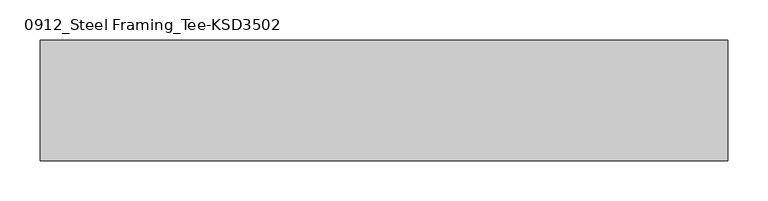
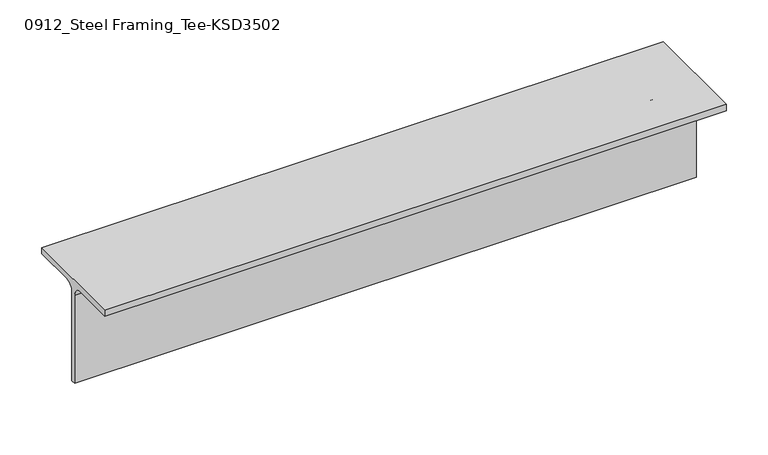
"""IFC4 building model written with IfcOpenShell, lengths in millimetres: member geometry, 0912_Steel Framing_Tee-KSD3502 : H_SB_ASB_CT-150x150x6.5x9."""

import ifcopenshell
import ifcopenshell.guid

model = None  # the IFC model being written
_history = None  # IfcOwnerHistory: only IFC2X3 demands one
_inside = {}  # id of a spatial element -> (the spatial element, [elements in it])
_under = {}  # id of a project, library or spatial element -> (it, [spatial elements below it])
_declared = {}  # id of a project -> (the project, [libraries it declares])
_typed = {}  # id of a type object -> (the type object, [elements of that type])
_made_of = {}  # id of a material, layer set ... -> (it, [elements and type objects made of it])


def new_model(schema):
    """Start an empty IFC model of exactly this schema.

    Asked for "IFC4X3", IfcOpenShell would pick the latest addendum, in which some entities
    have other attributes; the version numbers below select the first issue.
    IFC2X3 requires an IfcOwnerHistory on every rooted entity: one is made here for all.
    """
    global model, _history
    if schema == "IFC4X3":
        model = ifcopenshell.file(schema_version=(4, 3, 0, 0))
    else:
        model = ifcopenshell.file(schema=schema)
    _inside.clear()
    _under.clear()
    _declared.clear()
    _typed.clear()
    _made_of.clear()
    _history = None
    if model.schema == "IFC2X3":
        org = make("IfcOrganization", Name="unknown")
        user = make(
            "IfcPersonAndOrganization",
            ThePerson=make("IfcPerson", FamilyName="unknown"),
            TheOrganization=org,
        )
        app = make(
            "IfcApplication",
            ApplicationDeveloper=org,
            Version="unknown",
            ApplicationFullName="unknown",
            ApplicationIdentifier="unknown",
        )
        _history = make(
            "IfcOwnerHistory",
            OwningUser=user,
            OwningApplication=app,
            ChangeAction="ADDED",
            CreationDate=0,
        )
    return model


def make(cls, **values):
    """One entity of the class cls with the attributes given. An attribute that is None is left unset."""
    return model.create_entity(
        cls, **{name: value for name, value in values.items() if value is not None}
    )


def rooted(cls, **values):
    """An entity with a GlobalId (a new one), such as an element, a storey or a relation."""
    return make(cls, GlobalId=ifcopenshell.guid.new(), OwnerHistory=_history, **values)


def si_unit(unit_type, name, prefix=None):
    """IfcSIUnit, for example si_unit("LENGTHUNIT", "METRE", prefix="MILLI")."""
    return make("IfcSIUnit", UnitType=unit_type, Prefix=prefix, Name=name)


def assignment(units):
    """IfcUnitAssignment: the units of a project."""
    return None if units is None else make("IfcUnitAssignment", Units=units)


def point(xyz):
    """IfcCartesianPoint."""
    return None if xyz is None else make("IfcCartesianPoint", Coordinates=xyz)


def direction(xyz):
    """IfcDirection."""
    return None if xyz is None else make("IfcDirection", DirectionRatios=xyz)


def frame(location, z_axis=None, x_axis=None):
    """IfcAxis2Placement3D, a coordinate frame: its origin and axes. An axis left out is left unset."""
    return make(
        "IfcAxis2Placement3D",
        Location=point(location),
        Axis=direction(z_axis),
        RefDirection=direction(x_axis),
    )


def frame_2d(location, x_axis=None):
    """IfcAxis2Placement2D, a coordinate frame in the plane: its origin and x axis."""
    return make(
        "IfcAxis2Placement2D", Location=point(location), RefDirection=direction(x_axis)
    )


def origin():
    """The frame at (0, 0, 0) with its axes left unset."""
    return frame((0.0, 0.0, 0.0))


def place(relative_to, where):
    """IfcLocalPlacement: puts the frame where relative to a parent placement (None: the world)."""
    return make(
        "IfcLocalPlacement", PlacementRelTo=relative_to, RelativePlacement=where
    )


def context(
    kind, dimensions, precision=None, world=None, true_north=None, identifier=None
):
    """IfcGeometricRepresentationContext, for example the 3D "Model" context."""
    return make(
        "IfcGeometricRepresentationContext",
        ContextIdentifier=identifier,
        ContextType=kind,
        CoordinateSpaceDimension=dimensions,
        Precision=precision,
        WorldCoordinateSystem=world,
        TrueNorth=true_north,
    )


def project(units=None, contexts=None):
    """IfcProject with its units and contexts."""
    return rooted(
        "IfcProject",
        Name="project",
        RepresentationContexts=contexts,
        UnitsInContext=assignment(units),
    )


def spatial(cls, under=None, at=None, **own):
    """A site, building, storey or space (cls), placed at a placement, below another one or the project."""
    s = rooted(cls, ObjectPlacement=at, **own)
    if under is not None:
        _under.setdefault(under.id(), (under, []))[1].append(s)
    return s


def polyline(points):
    """IfcPolyline through the points."""
    return make("IfcPolyline", Points=[point(p) for p in points])


def circle_curve(where, radius):
    """IfcCircle in the frame where."""
    return make("IfcCircle", Position=where, Radius=radius)


def trimmed(basis, trim1, trim2, sense, master):
    """IfcTrimmedCurve: the piece of a basis curve between two trims."""
    return make(
        "IfcTrimmedCurve",
        BasisCurve=basis,
        Trim1=trim1,
        Trim2=trim2,
        SenseAgreement=sense,
        MasterRepresentation=master,
    )


def segment(curve, same_sense, transition):
    """IfcCompositeCurveSegment."""
    return make(
        "IfcCompositeCurveSegment",
        Transition=transition,
        SameSense=same_sense,
        ParentCurve=curve,
    )


def composite_curve(segments, self_intersect=None):
    """IfcCompositeCurve: segments joined end to end."""
    return make("IfcCompositeCurve", Segments=segments, SelfIntersect=self_intersect)


def outline(outer, holes=None, kind="AREA"):
    """IfcArbitraryClosedProfileDef: a profile drawn as a closed curve; with holes, ...WithVoids."""
    if holes is None:
        return make("IfcArbitraryClosedProfileDef", ProfileType=kind, OuterCurve=outer)
    return make(
        "IfcArbitraryProfileDefWithVoids",
        ProfileType=kind,
        OuterCurve=outer,
        InnerCurves=holes,
    )


def extrude(swept, where, along, depth):
    """IfcExtrudedAreaSolid: the profile swept, set in the frame where, extruded along a direction by depth."""
    return make(
        "IfcExtrudedAreaSolid",
        SweptArea=swept,
        Position=where,
        ExtrudedDirection=direction(along),
        Depth=depth,
    )


def shape(context_of_items, identifier, shape_type, items):
    """IfcShapeRepresentation: the items that make up one representation, for example the "Body"."""
    return make(
        "IfcShapeRepresentation",
        ContextOfItems=context_of_items,
        RepresentationIdentifier=identifier,
        RepresentationType=shape_type,
        Items=items,
    )


def source(mapping_origin, context_of_items, identifier, shape_type, items):
    """IfcRepresentationMap: a shape defined once, which mapped items show again and again."""
    return make(
        "IfcRepresentationMap",
        MappingOrigin=mapping_origin,
        MappedRepresentation=shape(context_of_items, identifier, shape_type, items),
    )


def transform(
    local_origin,
    x_axis=None,
    y_axis=None,
    z_axis=None,
    scale=None,
    scale2=None,
    scale3=None,
    uniform=True,
):
    """IfcCartesianTransformationOperator3D, or its non-uniform kind. x_axis, y_axis, z_axis: its Axis1, 2, 3."""
    if uniform:
        return make(
            "IfcCartesianTransformationOperator3D",
            Axis1=direction(x_axis),
            Axis2=direction(y_axis),
            LocalOrigin=point(local_origin),
            Scale=scale,
            Axis3=direction(z_axis),
        )
    return make(
        "IfcCartesianTransformationOperator3DnonUniform",
        Axis1=direction(x_axis),
        Axis2=direction(y_axis),
        LocalOrigin=point(local_origin),
        Scale=scale,
        Axis3=direction(z_axis),
        Scale2=scale2,
        Scale3=scale3,
    )


def mapped(mapping_source, mapping_target):
    """IfcMappedItem: shows the shape of a source again, moved by a transform."""
    return make(
        "IfcMappedItem", MappingSource=mapping_source, MappingTarget=mapping_target
    )


def made_of(thing, what):
    """Note that an element or type object is made of a material, layer set ...; save() writes the relation."""
    if what is not None:
        _made_of.setdefault(what.id(), (what, []))[1].append(thing)
    return thing


def element(
    cls,
    number,
    at=None,
    inside=None,
    cuts=None,
    type_object=None,
    material=None,
    context=None,
    identifier="Body",
    shape_type=None,
    held_by="IfcProductDefinitionShape",
    body=None,
    shapes=None,
    **own,
):
    """One element of the class cls, such as IfcWall. Its Tag is "e" and its number.

    at: its placement. inside: the storey or other place that contains it. cuts: it is an
    opening in that element (IfcRelVoidsElement). A single representation is given by context,
    identifier, shape_type and body (its items); several are given by shapes. held_by: the class
    of the entity that holds the representations. save() writes the other relations.
    """
    e = rooted(cls, Tag="e%d" % number, ObjectPlacement=at, **own)
    if body is not None:
        shapes = [shape(context, identifier, shape_type, body)]
    if shapes is not None:
        e.Representation = make(held_by, Representations=shapes)
    if inside is not None:
        _inside.setdefault(inside.id(), (inside, []))[1].append(e)
    if cuts is not None:
        rooted(
            "IfcRelVoidsElement", RelatingBuildingElement=cuts, RelatedOpeningElement=e
        )
    if type_object is not None:
        _typed.setdefault(type_object.id(), (type_object, []))[1].append(e)
    return made_of(e, material)


def aggregate(whole, parts):
    """IfcRelAggregates: a whole, such as a stair, and the parts it consists of."""
    return rooted("IfcRelAggregates", RelatingObject=whole, RelatedObjects=parts)


def save(model, path):
    """Write the relations noted so far, then the file.

    IfcRelAggregates (storeys below a building ...), IfcRelContainedInSpatialStructure (elements
    in a storey), IfcRelDefinesByType, IfcRelAssociatesMaterial and IfcRelDeclares: one each for
    every whole, place, type object, material and project.
    """
    for whole, parts in _under.values():
        aggregate(whole, parts)
    for where, things in _inside.values():
        rooted(
            "IfcRelContainedInSpatialStructure",
            RelatedElements=things,
            RelatingStructure=where,
        )
    for kind, things in _typed.values():
        rooted("IfcRelDefinesByType", RelatedObjects=things, RelatingType=kind)
    for what, things in _made_of.values():
        rooted("IfcRelAssociatesMaterial", RelatedObjects=things, RelatingMaterial=what)
    for by, libraries in _declared.values():
        rooted("IfcRelDeclares", RelatingContext=by, RelatedDefinitions=libraries)
    model.write(path)


def member_0912_steel_framing_tee_ksd3502_96588f7a(model_context):
    return source(origin(), model_context, "Body", "SweptSolid", [
        extrude(outline(composite_curve([segment(polyline([(-75.0, 75.0), (75.0, 75.0), (75.0, 66.0), (16.25, 66.0)]), True, "CONTINUOUS"), segment(trimmed(circle_curve(frame_2d((16.25, 53.0)), 13.0), [point((16.25, 66.0))], [point((3.25, 53.0))], True, "CARTESIAN"), True, "CONTINUOUS"), segment(polyline([(3.25, 53.0), (3.25, -75.0), (-3.25, -75.0), (-3.25, 53.0)]), True, "CONTINUOUS"), segment(trimmed(circle_curve(frame_2d((-16.25, 53.0)), 13.0), [point((-3.25, 53.0))], [point((-16.25, 66.0))], True, "CARTESIAN"), True, "CONTINUOUS"), segment(polyline([(-16.25, 66.0), (-75.0, 66.0), (-75.0, 75.0)]), True, "CONTINUOUS")], self_intersect=False)), frame((-356.1, 0.0, 0.0), z_axis=(1.0, 0.0, 0.0), x_axis=(0.0, 1.0, 0.0)), (0.0, 0.0, 1.0), 856.1),
    ])


if __name__ == "__main__":
    model = new_model("IFC4")
    model_context = context("Model", 3, world=origin())
    ifc_project = project(units=[si_unit("LENGTHUNIT", "METRE", prefix="MILLI")], contexts=[model_context])
    site = spatial("IfcSite", under=ifc_project)
    building = spatial("IfcBuilding", under=site)
    placement = place(None, origin())
    member_0912_steel_framing_tee_ksd3502_shape = member_0912_steel_framing_tee_ksd3502_96588f7a(model_context)
    element("IfcMember", 1, ObjectType="0912_Steel Framing_Tee-KSD3502 : H_SB_ASB_CT-150x150x6.5x9", at=placement, inside=building, context=model_context, shape_type="MappedRepresentation", body=[
        mapped(member_0912_steel_framing_tee_ksd3502_shape, transform((0.0, 0.0, 0.0), x_axis=(1.0, 0.0, 0.0), y_axis=(0.0, 1.0, 0.0), z_axis=(0.0, 0.0, 1.0))),
    ])
    save(model, "model.ifc")

# Revit data of these elements
# Type "0912_Steel Framing_Tee-KSD3502 : H_SB_ASB_CT-150x150x6.5x9"
#   H_WM Code_1 = "S01AA003-00001 | Main Steel Structure Fabrication Work | Shelter/Building | Light Steel - Standard (30KG/M>Weight) | Material: (   )"
#   H_WM Code_2 = "S03AA029-00001 | Main Steel Structure Erection Work | Shelter/Building | Light Steel (30KG/M>Weight) | Material: (   )"
#   H_WM Code_3 = "S01AA010-00001 | Main Steel Structure Fabrication Work | Shelter/Building | Steel Painting/Coating | for Non-Fireproofed Steel Surface, Surface Preparation, Primer, Second & Final Coat | Material: (   )"
#   H_Q'ty Cal Type Tag = "SB-Q2"
#   Width = 15.0 cm
#   Web Thickness = 0.65 cm
#   Web Fillet = 1.3 cm
#   Section Area = 23.39 cm²
#   Perimeter = 0.60 m²/m
#   Nominal Weight = 18.40 kgf/m
#   Height = 15.0 cm
#   Flange Thickness = 0.9 cm
#   Centroid Vertical = 7.5 cm
#   Centroid Horizontal = 7.5 cm
#   Length [instance default] = 1.5000 m
#   Structural Material [instance default] = Steel, 45-345
#   Warping Constant = (empty or 0)
#   Torsional Moment of Inertia = 0
#   Section Name Key = ""
#   Plastic Modulus weak axis = 0
#   Plastic Modulus strong axis = 0
#   Moment of Inertia weak axis = 0
#   Moment of Inertia strong axis = 0
#   Elastic Modulus weak axis = 0
#   Elastic Modulus strong axis = 0
#   Bolt Spacing = 0
#   Assembly Code = ""
# Element 1 (IfcMember, "0912_Steel Framing_Tee-KSD3502 : H_SB_ASB_CT-150x150x6.5x9")
#   Structural Material = none
# Materials
#   "Steel, 45-345": class "Metal", colour RGB 189 187 185, transparency 0, Description = "Steel 345 MPa", Cost = 0
